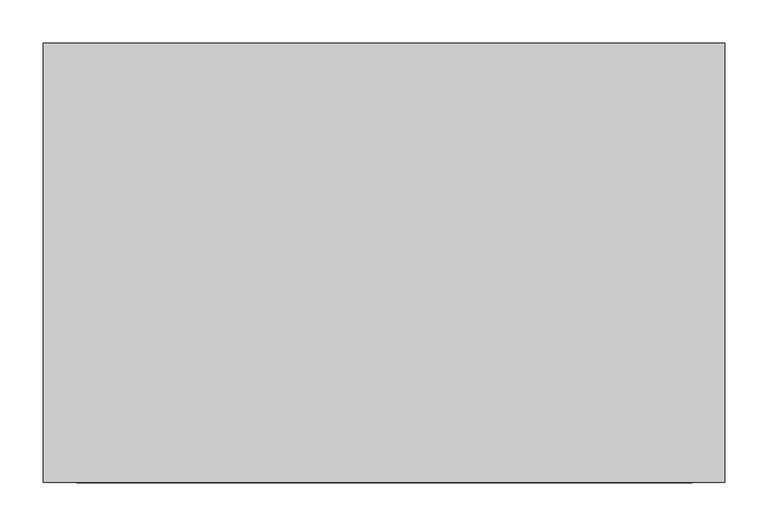
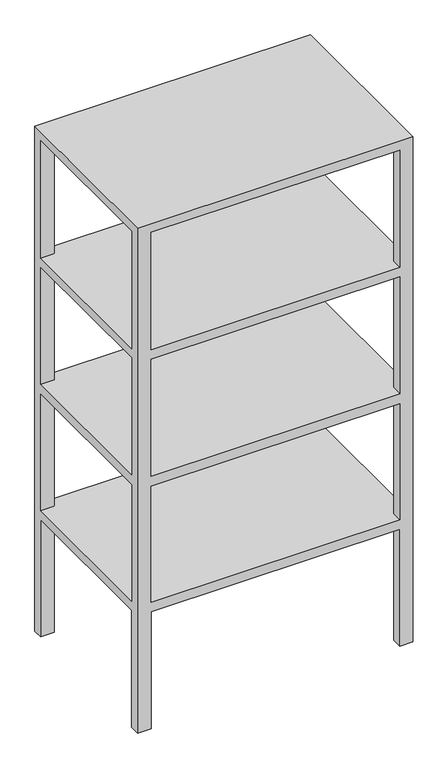
"""IFC4 building model written with IfcOpenShell, lengths in millimetres: furniture geometry, Preserved mushrrom shelf2 : Preserved mushrrom shelf."""

from ifc_helpers import new_model, si_unit, origin, place, context, project, spatial, faceted_brep, source, transform, mapped, element, save


def furniture_13ba74b9(model_context):
    return source(origin(), model_context, "Body", "Brep", [
        faceted_brep([(10489.488508, 2172.9615366, 1524.0), (10489.488508, 2680.9615366, 1524.0), (9702.088508, 2680.9615366, 1524.0), (9702.088508, 2172.9615366, 1524.0), (10489.488508, 2172.9615366, 0.0), (10452.1087778, 2172.9615366, 0.0), (10452.1087778, 2201.9838057, 0.0), (10489.488508, 2201.9838057, 0.0), (10452.1087778, 2680.9615366, 0.0), (10489.488508, 2680.9615366, 0.0), (10489.488508, 2652.0377422, 0.0), (10452.1087778, 2652.0377422, 0.0), (9740.9087778, 2172.9615366, 0.0), (9702.088508, 2172.9615366, 0.0), (9702.088508, 2201.9838057, 0.0), (9740.9087778, 2201.9838057, 0.0), (9702.088508, 2652.0377422, 0.0), (9702.088508, 2680.9615366, 0.0), (9740.9087778, 2680.9615366, 0.0), (9740.9087778, 2652.0377422, 0.0), (9740.9087778, 2172.9615366, 353.3332002), (10452.1087778, 2172.9615366, 353.3332002), (9740.9087778, 2172.9615366, 1497.6781444), (10452.1087778, 2172.9615366, 1497.6781444), (10452.1087778, 2172.9615366, 1143.0), (9740.9087778, 2172.9615366, 1143.0), (9740.9087778, 2172.9615366, 1114.8196695), (10452.1087778, 2172.9615366, 1114.8196695), (10452.1087778, 2172.9615366, 762.0), (9740.9087778, 2172.9615366, 762.0), (9740.9087778, 2172.9615366, 731.9611947), (10452.1087778, 2172.9615366, 731.9611947), (10452.1087778, 2172.9615366, 381.0), (9740.9087778, 2172.9615366, 381.0), (9702.088508, 2652.0377422, 353.3332002), (9702.088508, 2201.9838057, 353.3332002), (9702.088508, 2652.0377422, 1497.6781444), (9702.088508, 2201.5559348, 1497.6781444), (9702.088508, 2201.5559348, 1143.0), (9702.088508, 2652.0377422, 1143.0), (9702.088508, 2652.0377422, 1114.8196695), (9702.088508, 2201.9838057, 1114.8196695), (9702.088508, 2201.9838057, 762.0), (9702.088508, 2652.0377422, 762.0), (9702.088508, 2652.0377422, 731.9611947), (9702.088508, 2201.9838057, 731.9611947), (9702.088508, 2201.9838057, 381.0), (9702.088508, 2652.0377422, 381.0), (10452.1087778, 2680.9615366, 353.3332002), (9740.9087778, 2680.9615366, 353.3332002), (10452.1087778, 2680.9615366, 1497.6781444), (9740.9087778, 2680.9615366, 1497.6781444), (9740.9087778, 2680.9615366, 1143.0), (10452.1087778, 2680.9615366, 1143.0), (10452.1087778, 2680.9615366, 1114.8196695), (9740.9087778, 2680.9615366, 1114.8196695), (9740.9087778, 2680.9615366, 762.0), (10452.1087778, 2680.9615366, 762.0), (10452.1087778, 2680.9615366, 731.9611947), (9740.9087778, 2680.9615366, 731.9611947), (9740.9087778, 2680.9615366, 381.0), (10452.1087778, 2680.9615366, 381.0), (10489.488508, 2201.9838057, 353.3332002), (10489.488508, 2652.0377422, 353.3332002), (10489.488508, 2201.9838057, 1497.6781444), (10489.488508, 2652.0377422, 1497.6781444), (10489.488508, 2652.0377422, 1143.0), (10489.488508, 2201.9838057, 1143.0), (10489.488508, 2201.9838057, 1114.8196695), (10489.488508, 2652.0377422, 1114.8196695), (10489.488508, 2652.0377422, 762.0), (10489.488508, 2201.9838057, 762.0), (10489.488508, 2201.9838057, 731.9611947), (10489.488508, 2652.0377422, 731.9611947), (10489.488508, 2652.0377422, 381.0), (10489.488508, 2201.9838057, 381.0), (9740.9087778, 2652.0377422, 1497.6781444), (10452.1087778, 2652.0377422, 1497.6781444), (10452.1087778, 2201.9838057, 1497.6781444), (9740.9087778, 2201.5559348, 1497.6781444), (9740.9087778, 2652.0377422, 1143.0), (9740.9087778, 2201.5559348, 1143.0), (10452.1087778, 2201.9838057, 1143.0), (10452.1087778, 2652.0377422, 1143.0), (9740.9087778, 2652.0377422, 1114.8196695), (10452.1087778, 2652.0377422, 1114.8196695), (10452.1087778, 2201.9838057, 1114.8196695), (9740.9087778, 2201.9838057, 1114.8196695), (9740.9087778, 2652.0377422, 762.0), (9740.9087778, 2201.9838057, 762.0), (10452.1087778, 2201.9838057, 762.0), (10452.1087778, 2652.0377422, 762.0), (9740.9087778, 2652.0377422, 731.9611947), (10452.1087778, 2652.0377422, 731.9611947), (10452.1087778, 2201.9838057, 731.9611947), (9740.9087778, 2201.9838057, 731.9611947), (9740.9087778, 2652.0377422, 381.0), (9740.9087778, 2201.9838057, 381.0), (10452.1087778, 2201.9838057, 381.0), (10452.1087778, 2652.0377422, 381.0), (9740.9087778, 2652.0377422, 353.3332002), (10452.1087778, 2652.0377422, 353.3332002), (10452.1087778, 2201.9838057, 353.3332002), (9740.9087778, 2201.9838057, 353.3332002)], [[[0, 1, 2, 3]], [[4, 5, 6, 7]], [[8, 9, 10, 11]], [[12, 13, 14, 15]], [[16, 17, 18, 19]], [[0, 3, 13, 12, 20, 21, 5, 4], [22, 23, 24, 25], [26, 27, 28, 29], [30, 31, 32, 33]], [[3, 2, 17, 16, 34, 35, 14, 13], [36, 37, 38, 39], [40, 41, 42, 43], [44, 45, 46, 47]], [[2, 1, 9, 8, 48, 49, 18, 17], [50, 51, 52, 53], [54, 55, 56, 57], [58, 59, 60, 61]], [[1, 0, 4, 7, 62, 63, 10, 9], [64, 65, 66, 67], [68, 69, 70, 71], [72, 73, 74, 75]], [[76, 51, 50, 77, 65, 64, 78, 23, 22, 79, 37, 36]], [[80, 39, 38, 81, 25, 24, 82, 67, 66, 83, 53, 52]], [[51, 76, 80, 52]], [[77, 50, 53, 83]], [[65, 77, 83, 66]], [[78, 64, 67, 82]], [[23, 78, 82, 24]], [[79, 22, 25, 81]], [[37, 79, 81, 38]], [[76, 36, 39, 80]], [[84, 55, 54, 85, 69, 68, 86, 27, 26, 87, 41, 40]], [[88, 43, 42, 89, 29, 28, 90, 71, 70, 91, 57, 56]], [[55, 84, 88, 56]], [[85, 54, 57, 91]], [[69, 85, 91, 70]], [[86, 68, 71, 90]], [[27, 86, 90, 28]], [[87, 26, 29, 89]], [[41, 87, 89, 42]], [[84, 40, 43, 88]], [[92, 59, 58, 93, 73, 72, 94, 31, 30, 95, 45, 44]], [[96, 47, 46, 97, 33, 32, 98, 75, 74, 99, 61, 60]], [[59, 92, 96, 60]], [[93, 58, 61, 99]], [[73, 93, 99, 74]], [[94, 72, 75, 98]], [[31, 94, 98, 32]], [[95, 30, 33, 97]], [[45, 95, 97, 46]], [[92, 44, 47, 96]], [[100, 49, 48, 101, 63, 62, 102, 21, 20, 103, 35, 34]], [[49, 100, 19, 18]], [[101, 48, 8, 11]], [[63, 101, 11, 10]], [[102, 62, 7, 6]], [[21, 102, 6, 5]], [[103, 20, 12, 15]], [[35, 103, 15, 14]], [[100, 34, 16, 19]]]),
    ])


if __name__ == "__main__":
    model = new_model("IFC4")
    model_context = context("Model", 3, world=origin())
    ifc_project = project(units=[si_unit("LENGTHUNIT", "METRE", prefix="MILLI")], contexts=[model_context])
    site = spatial("IfcSite", under=ifc_project)
    building = spatial("IfcBuilding", under=site)
    placement = place(None, origin())
    furniture_shape = furniture_13ba74b9(model_context)
    element("IfcFurniture", 1, ObjectType="Preserved mushrrom shelf2 : Preserved mushrrom shelf", at=placement, inside=building, context=model_context, shape_type="MappedRepresentation", body=[
        mapped(furniture_shape, transform((0.0, 0.0, 0.0), x_axis=(1.0, 0.0, 0.0), y_axis=(0.0, 1.0, 0.0), z_axis=(0.0, 0.0, 1.0))),
    ])
    save(model, "model.ifc")

# Revit data of these elements
# Element 1 (IfcFurniture, "Preserved mushrrom shelf2 : Preserved mushrrom shelf")
#   Materials on its faces: "food"
# Materials
#   "food": class "Glass", colour RGB 233 233 233, transparency 0, Description = "Soda Lime Glass", Cost = 0
